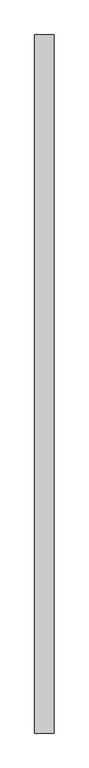
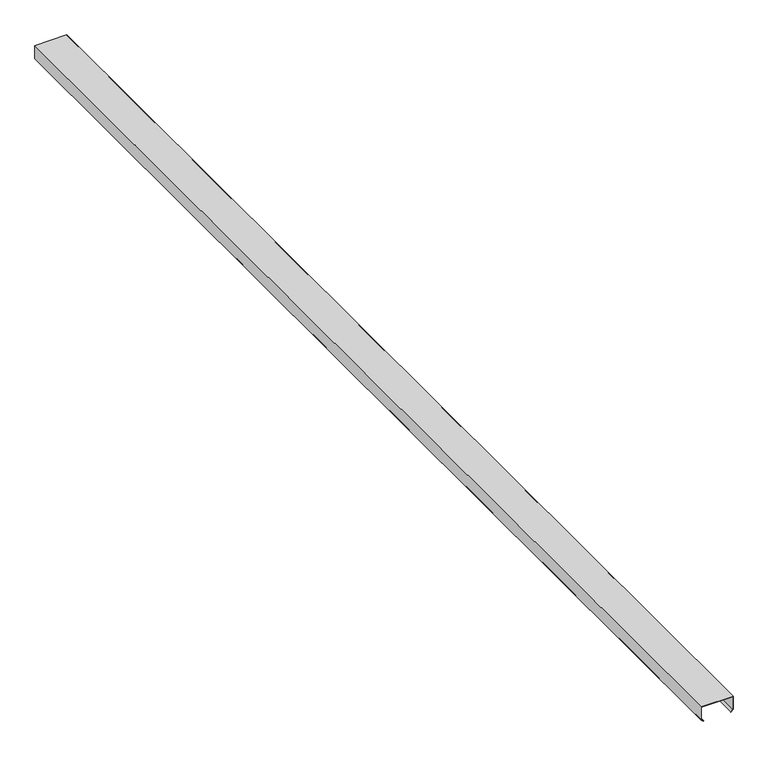
"""IFC4 building model written with IfcOpenShell, lengths in millimetres: proxy geometry, Generic Models 7:Generic Models 1:1:Generic Models 1:1 : Generic Models 7:Generic Models 1:337419:19 : Generic Models 7:Generic Models 1:1:Generic Models 1:1 : Generic Models 7:Generic Models 1:337419:306201."""

from ifc_helpers import new_model, si_unit, frame, origin, place, context, project, spatial, polyline, outline, extrude, source, transform, mapped, element, save


def generic_models_2c2944e3(model_context):
    return source(origin(), model_context, "Body", "SweptSolid", [
        extrude(outline(polyline([(6128.940625, 579307.711724), (6128.940625, 579104.511724), (6040.040625, 579104.511724), (6027.7955211, 579119.1048707), (6029.9236883, 579120.890615), (6041.336086, 579107.289849), (6126.1625, 579107.289849), (6126.1625, 579304.933599), (6041.336086, 579304.933599), (6029.9236883, 579291.3328331), (6027.7955211, 579293.1185774), (6040.040625, 579307.711724), (6128.940625, 579307.711724)])), frame((0.0, -581258.1163841, 0.0), z_axis=(0.0, 1.0, 0.0), x_axis=(0.0, 0.0, 1.0)), (0.0, 0.0, 1.0), 7315.2),
    ])


if __name__ == "__main__":
    model = new_model("IFC4")
    model_context = context("Model", 3, world=origin())
    ifc_project = project(units=[si_unit("LENGTHUNIT", "METRE", prefix="MILLI")], contexts=[model_context])
    site = spatial("IfcSite", under=ifc_project)
    building = spatial("IfcBuilding", under=site)
    placement = place(None, origin())
    generic_models_shape = generic_models_2c2944e3(model_context)
    element("IfcBuildingElementProxy", 1, Name="Generic Models 7:Generic Models 1:1:Generic Models 1:1 : Generic Models 7:Generic Models 1:337419:19 : Generic Models 7:Generic Models 1:1:Generic Models 1:1 : Generic Models 7:Generic Models 1:337419:306201", ObjectType="Generic Models 7:Generic Models 1:1:Generic Models 1:1 : Generic Models 7:Generic Models 1:337419:19 : Generic Models 7:Generic Models 1:1:Generic Models 1:1 : Generic Models 7:Generic Models 1:337419:306201", at=placement, inside=building, context=model_context, shape_type="MappedRepresentation", body=[
        mapped(generic_models_shape, transform((0.0, 0.0, 0.0), x_axis=(1.0, 0.0, 0.0), y_axis=(0.0, 1.0, 0.0), z_axis=(0.0, 0.0, 1.0))),
    ])
    save(model, "model.ifc")

# Revit data of these elements
# Type "Generic Models 7:Generic Models 1:1:Generic Models 1:1 : Generic Models 7:Generic Models 1:337419:19 : Generic Models 7:Generic Models 1:1:Generic Models 1:1 : Generic Models 7:Generic Models 1:337419:306201"
#   NameOverride = "Generic Models 7:Generic Models 1:1:Generic Models 1:1 : Generic Models 7:Generic Models 1:337419:306201"
#   ObjectTypeOverride = "Generic Models 1:1 : Generic Models 7:Generic Models 1:337419"
#   Reference = "Generic Models 1"
#   Tag = "306201"
# Element 1 (IfcBuildingElementProxy, "Generic Models 7:Generic Models 1:1:Generic Models 1:1 : Generic Models 7:Generic Models 1:337419:19 : Generic Models 7:Generic Models 1:1:Generic Models 1:1 : Generic Models 7:Generic Models 1:337419:306201")
#   Materials on its faces: "'ZEE' SECTION (8.0x3.5Z - SEE STRUCT. DWGS)"
# Materials
#   "'ZEE' SECTION (8.0x3.5Z - SEE STRUCT. DWGS)": class "Unassigned", colour RGB 210 209 208, transparency 0, Keynote = "M05121300.02", Cost = 0
